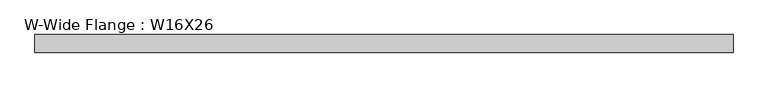
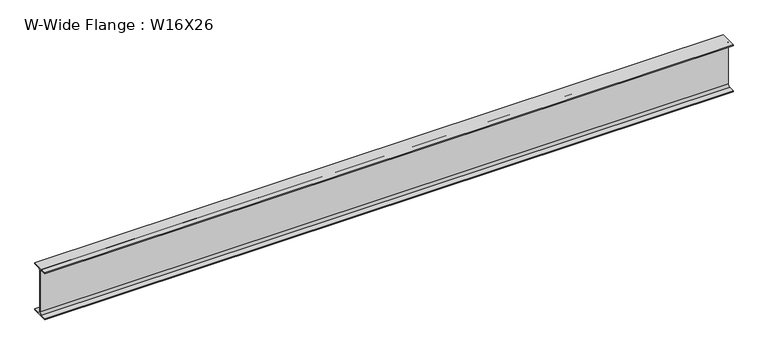
"""IFC4 building model written with IfcOpenShell, lengths in millimetres: beam geometry, W-Wide Flange : W16X26."""

from ifc_helpers import new_model, si_unit, point, frame, frame_2d, origin, place, context, project, spatial, polyline, circle_curve, trimmed, segment, composite_curve, outline, extrude, source, transform, mapped, element, save


def w_wide_flange_w16x26_d3961c21(model_context):
    return source(origin(), model_context, "Body", "SweptSolid", [
        extrude(outline(composite_curve([segment(polyline([(69.85, -190.627), (69.85, -199.39), (-69.85, -199.39), (-69.85, -190.627), (-21.3995, -190.627)]), True, "CONTINUOUS"), segment(trimmed(circle_curve(frame_2d((-21.3995, -172.4025)), 18.2245), [point((-21.3995, -190.627))], [point((-3.175, -172.4025))], True, "CARTESIAN"), True, "CONTINUOUS"), segment(polyline([(-3.175, -172.4025), (-3.175, 172.4025)]), True, "CONTINUOUS"), segment(trimmed(circle_curve(frame_2d((-21.3995, 172.4025)), 18.2245), [point((-3.175, 172.4025))], [point((-21.3995, 190.627))], True, "CARTESIAN"), True, "CONTINUOUS"), segment(polyline([(-21.3995, 190.627), (-69.85, 190.627), (-69.85, 199.39), (69.85, 199.39), (69.85, 190.627), (21.3995, 190.627)]), True, "CONTINUOUS"), segment(trimmed(circle_curve(frame_2d((21.3995, 172.4025)), 18.2245), [point((21.3995, 190.627))], [point((3.175, 172.4025))], True, "CARTESIAN"), True, "CONTINUOUS"), segment(polyline([(3.175, 172.4025), (3.175, -172.4025)]), True, "CONTINUOUS"), segment(trimmed(circle_curve(frame_2d((21.3995, -172.4025)), 18.2245), [point((3.175, -172.4025))], [point((21.3995, -190.627))], True, "CARTESIAN"), True, "CONTINUOUS"), segment(polyline([(21.3995, -190.627), (69.85, -190.627)]), True, "CONTINUOUS")], self_intersect=False)), frame((-2768.6, 0.0, 0.0), z_axis=(1.0, 0.0, 0.0), x_axis=(0.0, 1.0, 0.0)), (0.0, 0.0, 1.0), 5537.2),
    ])


if __name__ == "__main__":
    model = new_model("IFC4")
    model_context = context("Model", 3, world=origin())
    ifc_project = project(units=[si_unit("LENGTHUNIT", "METRE", prefix="MILLI")], contexts=[model_context])
    site = spatial("IfcSite", under=ifc_project)
    building = spatial("IfcBuilding", under=site)
    placement = place(None, origin())
    w_wide_flange_w16x26_shape = w_wide_flange_w16x26_d3961c21(model_context)
    element("IfcBeam", 1, ObjectType="W-Wide Flange : W16X26", at=placement, inside=building, context=model_context, shape_type="MappedRepresentation", body=[
        mapped(w_wide_flange_w16x26_shape, transform((0.0, 0.0, 0.0), x_axis=(1.0, 0.0, 0.0), y_axis=(0.0, 1.0, 0.0), z_axis=(0.0, 0.0, 1.0))),
    ])
    save(model, "model.ifc")

# Revit data of these elements
# Type "W-Wide Flange : W16X26"
#   Assembly Code = "B10"
#   W = 26
#   Length [instance default] = 5' - 0"
#   bf = 0' - 5 1/2"
#   d = 1' - 3.7"
#   k = 0' - 1 1/16"
#   k2 = 0' - 0.7175"
#   tf = 0' - 0.345"
#   tw = 0' - 0 1/4"
#   A = 0.0533333 SF
#   Structural Material [instance default] = Steel ASTM A992
# Element 1 (IfcBeam, "W-Wide Flange : W16X26")
#   Structural Material = Steel ASTM A36
#   Materials on its faces: "Steel ASTM A36"
# Materials
#   "Steel ASTM A992": class "Metal", colour RGB 199 199 199, transparency 0, Description = "Structural steel 50ksi", Cost = 0
#   "Steel ASTM A36": class "Metal", colour RGB 199 199 199, transparency 0, Description = "Structural steel, ASTM A36 Grade B, mill finish", Cost = 0
